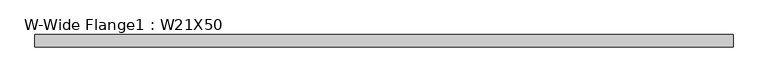
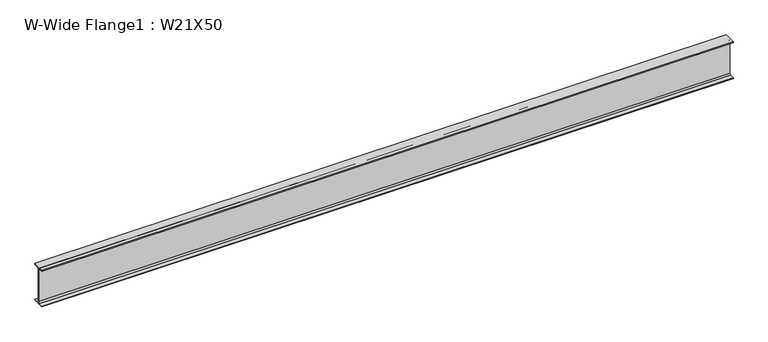
"""IFC4 building model written with IfcOpenShell, lengths in millimetres: beam geometry, W-Wide Flange1 : W21X50."""

from ifc_helpers import new_model, si_unit, point, frame, frame_2d, origin, place, context, project, spatial, polyline, circle_curve, trimmed, segment, composite_curve, outline, extrude, source, transform, mapped, element, save


def w_wide_flange1_w21x50_217575f8(model_context):
    return source(origin(), model_context, "Body", "SweptSolid", [
        extrude(outline(composite_curve([segment(polyline([(82.931, -250.571), (82.931, -264.16), (-82.931, -264.16), (-82.931, -250.571), (-22.987, -250.571)]), True, "CONTINUOUS"), segment(trimmed(circle_curve(frame_2d((-22.987, -232.41)), 18.161), [point((-22.987, -250.571))], [point((-4.826, -232.41))], True, "CARTESIAN"), True, "CONTINUOUS"), segment(polyline([(-4.826, -232.41), (-4.826, 232.41)]), True, "CONTINUOUS"), segment(trimmed(circle_curve(frame_2d((-22.987, 232.41)), 18.161), [point((-4.826, 232.41))], [point((-22.987, 250.571))], True, "CARTESIAN"), True, "CONTINUOUS"), segment(polyline([(-22.987, 250.571), (-82.931, 250.571), (-82.931, 264.16), (82.931, 264.16), (82.931, 250.571), (22.987, 250.571)]), True, "CONTINUOUS"), segment(trimmed(circle_curve(frame_2d((22.987, 232.41)), 18.161), [point((22.987, 250.571))], [point((4.826, 232.41))], True, "CARTESIAN"), True, "CONTINUOUS"), segment(polyline([(4.826, 232.41), (4.826, -232.41)]), True, "CONTINUOUS"), segment(trimmed(circle_curve(frame_2d((22.987, -232.41)), 18.161), [point((4.826, -232.41))], [point((22.987, -250.571))], True, "CARTESIAN"), True, "CONTINUOUS"), segment(polyline([(22.987, -250.571), (82.931, -250.571)]), True, "CONTINUOUS")], self_intersect=False)), frame((-4705.6575337, 0.0, 0.0), z_axis=(1.0, 0.0, 0.0), x_axis=(0.0, 1.0, 0.0)), (0.0, 0.0, 1.0), 9411.3150674),
    ])


if __name__ == "__main__":
    model = new_model("IFC4")
    model_context = context("Model", 3, world=origin())
    ifc_project = project(units=[si_unit("LENGTHUNIT", "METRE", prefix="MILLI")], contexts=[model_context])
    site = spatial("IfcSite", under=ifc_project)
    building = spatial("IfcBuilding", under=site)
    placement = place(None, origin())
    w_wide_flange1_w21x50_shape = w_wide_flange1_w21x50_217575f8(model_context)
    element("IfcBeam", 1, ObjectType="W-Wide Flange1 : W21X50", at=placement, inside=building, context=model_context, shape_type="MappedRepresentation", body=[
        mapped(w_wide_flange1_w21x50_shape, transform((0.0, 0.0, 0.0), x_axis=(1.0, 0.0, 0.0), y_axis=(0.0, 1.0, 0.0), z_axis=(0.0, 0.0, 1.0))),
    ])
    save(model, "model.ifc")

# Revit data of these elements
# Type "W-Wide Flange1 : W21X50"
#   Assembly Code = "B10"
#   W = 50
#   Start Extension Calculation [instance default] = 10' - 0"
#   Start Extension [instance default] = -0' - 0 1/2"
#   End Extension Calculation [instance default] = 10' - 0"
#   End Extension [instance default] = -0' - 0 1/2"
#   Length [instance default] = 5' - 0"
#   bf = 0' - 6.53"
#   d = 1' - 8.8"
#   k = 0' - 1 1/4"
#   k2 = 0' - 0.715"
#   tf = 0' - 0.535"
#   tw = 0' - 0.38"
#   A = 0.102083 SF
#   Structural Material [instance default] = Metal - Steel - ASTM A992
# Element 1 (IfcBeam, "W-Wide Flange1 : W21X50")
#   Materials on its faces: "Metal - Steel - ASTM A992"
# Materials
#   "Metal - Steel - ASTM A992": class "Metal", colour RGB 199 199 199, transparency 0
